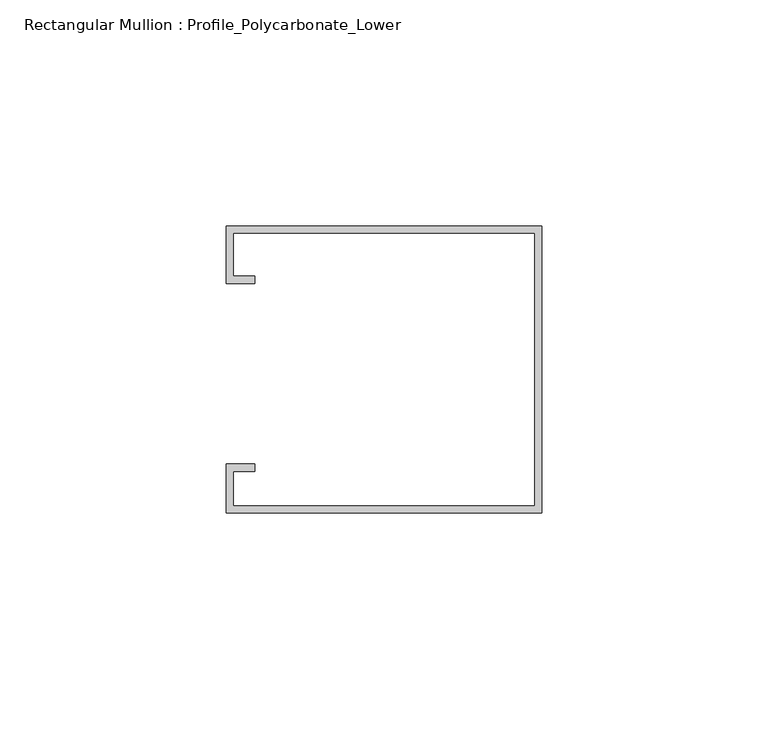
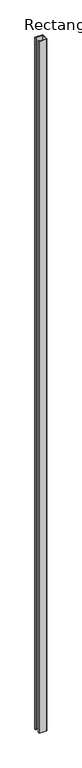
"""IFC4 building model written with IfcOpenShell, lengths in millimetres: member geometry, Rectangular Mullion : Profile_Polycarbonate_Lower."""

from ifc_helpers import new_model, si_unit, frame, origin, place, context, project, spatial, polyline, outline, extrude, source, transform, mapped, element, save


def rectangular_mullion_profile_polycarbonate_lower_94622d10(model_context):
    return source(origin(), model_context, "Body", "SweptSolid", [
        extrude(outline(polyline([(0.0, 32.7), (0.0, -30.8), (-69.85, -30.8), (-69.85, -20.0), (-63.5, -20.0), (-63.5, -21.5875), (-68.2625, -21.5875), (-68.2625, -29.2125), (-1.5875, -29.2125), (-1.5875, 31.1125), (-68.2625, 31.1125), (-68.2625, 21.5875), (-63.5, 21.5875), (-63.5, 20.0), (-69.85, 20.0), (-69.85, 32.7), (0.0, 32.7)])), frame((0.0, 0.0, -6550.025), z_axis=(0.0, 0.0, 1.0), x_axis=(1.0, 0.0, 0.0)), (0.0, 0.0, 1.0), 6550.025),
    ])


if __name__ == "__main__":
    model = new_model("IFC4")
    model_context = context("Model", 3, world=origin())
    ifc_project = project(units=[si_unit("LENGTHUNIT", "METRE", prefix="MILLI")], contexts=[model_context])
    site = spatial("IfcSite", under=ifc_project)
    building = spatial("IfcBuilding", under=site)
    placement = place(None, origin())
    rectangular_mullion_profile_polycarbonate_lower_shape = rectangular_mullion_profile_polycarbonate_lower_94622d10(model_context)
    element("IfcMember", 1, ObjectType="Rectangular Mullion : Profile_Polycarbonate_Lower", at=placement, inside=building, context=model_context, shape_type="MappedRepresentation", body=[
        mapped(rectangular_mullion_profile_polycarbonate_lower_shape, transform((0.0, 0.0, 0.0), x_axis=(1.0, 0.0, 0.0), y_axis=(0.0, 1.0, 0.0), z_axis=(0.0, 0.0, 1.0))),
    ])
    save(model, "model.ifc")

# Revit data of these elements
# Type "Rectangular Mullion : Profile_Polycarbonate_Lower"
#   built-in parameter 1007322 = 0.208333 (stored number, unit not read)
#   built-in parameter 1007321 = 0 (stored number, unit not read)
#   built-in parameter 1007320 = 0.00520833 (stored number, unit not read)
